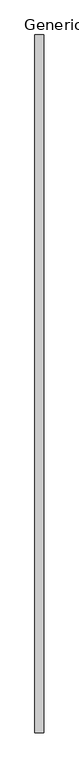
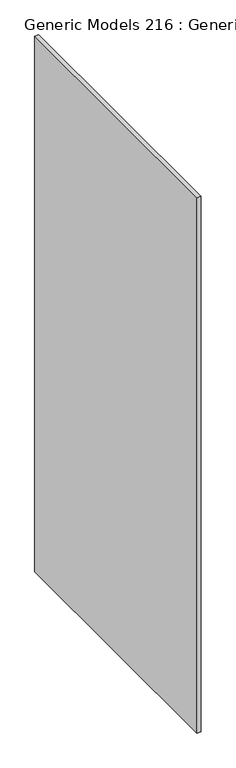
"""IFC4 building model written with IfcOpenShell, lengths in millimetres: proxy geometry, Generic Models 216 : Generic Models 1."""

import ifcopenshell
import ifcopenshell.guid

model = None  # the IFC model being written
_history = None  # IfcOwnerHistory: only IFC2X3 demands one
_inside = {}  # id of a spatial element -> (the spatial element, [elements in it])
_under = {}  # id of a project, library or spatial element -> (it, [spatial elements below it])
_declared = {}  # id of a project -> (the project, [libraries it declares])
_typed = {}  # id of a type object -> (the type object, [elements of that type])
_made_of = {}  # id of a material, layer set ... -> (it, [elements and type objects made of it])


def new_model(schema):
    """Start an empty IFC model of exactly this schema.

    Asked for "IFC4X3", IfcOpenShell would pick the latest addendum, in which some entities
    have other attributes; the version numbers below select the first issue.
    IFC2X3 requires an IfcOwnerHistory on every rooted entity: one is made here for all.
    """
    global model, _history
    if schema == "IFC4X3":
        model = ifcopenshell.file(schema_version=(4, 3, 0, 0))
    else:
        model = ifcopenshell.file(schema=schema)
    _inside.clear()
    _under.clear()
    _declared.clear()
    _typed.clear()
    _made_of.clear()
    _history = None
    if model.schema == "IFC2X3":
        org = make("IfcOrganization", Name="unknown")
        user = make(
            "IfcPersonAndOrganization",
            ThePerson=make("IfcPerson", FamilyName="unknown"),
            TheOrganization=org,
        )
        app = make(
            "IfcApplication",
            ApplicationDeveloper=org,
            Version="unknown",
            ApplicationFullName="unknown",
            ApplicationIdentifier="unknown",
        )
        _history = make(
            "IfcOwnerHistory",
            OwningUser=user,
            OwningApplication=app,
            ChangeAction="ADDED",
            CreationDate=0,
        )
    return model


def make(cls, **values):
    """One entity of the class cls with the attributes given. An attribute that is None is left unset."""
    return model.create_entity(
        cls, **{name: value for name, value in values.items() if value is not None}
    )


def rooted(cls, **values):
    """An entity with a GlobalId (a new one), such as an element, a storey or a relation."""
    return make(cls, GlobalId=ifcopenshell.guid.new(), OwnerHistory=_history, **values)


def si_unit(unit_type, name, prefix=None):
    """IfcSIUnit, for example si_unit("LENGTHUNIT", "METRE", prefix="MILLI")."""
    return make("IfcSIUnit", UnitType=unit_type, Prefix=prefix, Name=name)


def assignment(units):
    """IfcUnitAssignment: the units of a project."""
    return None if units is None else make("IfcUnitAssignment", Units=units)


def point(xyz):
    """IfcCartesianPoint."""
    return None if xyz is None else make("IfcCartesianPoint", Coordinates=xyz)


def direction(xyz):
    """IfcDirection."""
    return None if xyz is None else make("IfcDirection", DirectionRatios=xyz)


def frame(location, z_axis=None, x_axis=None):
    """IfcAxis2Placement3D, a coordinate frame: its origin and axes. An axis left out is left unset."""
    return make(
        "IfcAxis2Placement3D",
        Location=point(location),
        Axis=direction(z_axis),
        RefDirection=direction(x_axis),
    )


def origin():
    """The frame at (0, 0, 0) with its axes left unset."""
    return frame((0.0, 0.0, 0.0))


def place(relative_to, where):
    """IfcLocalPlacement: puts the frame where relative to a parent placement (None: the world)."""
    return make(
        "IfcLocalPlacement", PlacementRelTo=relative_to, RelativePlacement=where
    )


def context(
    kind, dimensions, precision=None, world=None, true_north=None, identifier=None
):
    """IfcGeometricRepresentationContext, for example the 3D "Model" context."""
    return make(
        "IfcGeometricRepresentationContext",
        ContextIdentifier=identifier,
        ContextType=kind,
        CoordinateSpaceDimension=dimensions,
        Precision=precision,
        WorldCoordinateSystem=world,
        TrueNorth=true_north,
    )


def project(units=None, contexts=None):
    """IfcProject with its units and contexts."""
    return rooted(
        "IfcProject",
        Name="project",
        RepresentationContexts=contexts,
        UnitsInContext=assignment(units),
    )


def spatial(cls, under=None, at=None, **own):
    """A site, building, storey or space (cls), placed at a placement, below another one or the project."""
    s = rooted(cls, ObjectPlacement=at, **own)
    if under is not None:
        _under.setdefault(under.id(), (under, []))[1].append(s)
    return s


def polyline(points):
    """IfcPolyline through the points."""
    return make("IfcPolyline", Points=[point(p) for p in points])


def outline(outer, holes=None, kind="AREA"):
    """IfcArbitraryClosedProfileDef: a profile drawn as a closed curve; with holes, ...WithVoids."""
    if holes is None:
        return make("IfcArbitraryClosedProfileDef", ProfileType=kind, OuterCurve=outer)
    return make(
        "IfcArbitraryProfileDefWithVoids",
        ProfileType=kind,
        OuterCurve=outer,
        InnerCurves=holes,
    )


def extrude(swept, where, along, depth):
    """IfcExtrudedAreaSolid: the profile swept, set in the frame where, extruded along a direction by depth."""
    return make(
        "IfcExtrudedAreaSolid",
        SweptArea=swept,
        Position=where,
        ExtrudedDirection=direction(along),
        Depth=depth,
    )


def shape(context_of_items, identifier, shape_type, items):
    """IfcShapeRepresentation: the items that make up one representation, for example the "Body"."""
    return make(
        "IfcShapeRepresentation",
        ContextOfItems=context_of_items,
        RepresentationIdentifier=identifier,
        RepresentationType=shape_type,
        Items=items,
    )


def source(mapping_origin, context_of_items, identifier, shape_type, items):
    """IfcRepresentationMap: a shape defined once, which mapped items show again and again."""
    return make(
        "IfcRepresentationMap",
        MappingOrigin=mapping_origin,
        MappedRepresentation=shape(context_of_items, identifier, shape_type, items),
    )


def transform(
    local_origin,
    x_axis=None,
    y_axis=None,
    z_axis=None,
    scale=None,
    scale2=None,
    scale3=None,
    uniform=True,
):
    """IfcCartesianTransformationOperator3D, or its non-uniform kind. x_axis, y_axis, z_axis: its Axis1, 2, 3."""
    if uniform:
        return make(
            "IfcCartesianTransformationOperator3D",
            Axis1=direction(x_axis),
            Axis2=direction(y_axis),
            LocalOrigin=point(local_origin),
            Scale=scale,
            Axis3=direction(z_axis),
        )
    return make(
        "IfcCartesianTransformationOperator3DnonUniform",
        Axis1=direction(x_axis),
        Axis2=direction(y_axis),
        LocalOrigin=point(local_origin),
        Scale=scale,
        Axis3=direction(z_axis),
        Scale2=scale2,
        Scale3=scale3,
    )


def mapped(mapping_source, mapping_target):
    """IfcMappedItem: shows the shape of a source again, moved by a transform."""
    return make(
        "IfcMappedItem", MappingSource=mapping_source, MappingTarget=mapping_target
    )


def made_of(thing, what):
    """Note that an element or type object is made of a material, layer set ...; save() writes the relation."""
    if what is not None:
        _made_of.setdefault(what.id(), (what, []))[1].append(thing)
    return thing


def element(
    cls,
    number,
    at=None,
    inside=None,
    cuts=None,
    type_object=None,
    material=None,
    context=None,
    identifier="Body",
    shape_type=None,
    held_by="IfcProductDefinitionShape",
    body=None,
    shapes=None,
    **own,
):
    """One element of the class cls, such as IfcWall. Its Tag is "e" and its number.

    at: its placement. inside: the storey or other place that contains it. cuts: it is an
    opening in that element (IfcRelVoidsElement). A single representation is given by context,
    identifier, shape_type and body (its items); several are given by shapes. held_by: the class
    of the entity that holds the representations. save() writes the other relations.
    """
    e = rooted(cls, Tag="e%d" % number, ObjectPlacement=at, **own)
    if body is not None:
        shapes = [shape(context, identifier, shape_type, body)]
    if shapes is not None:
        e.Representation = make(held_by, Representations=shapes)
    if inside is not None:
        _inside.setdefault(inside.id(), (inside, []))[1].append(e)
    if cuts is not None:
        rooted(
            "IfcRelVoidsElement", RelatingBuildingElement=cuts, RelatedOpeningElement=e
        )
    if type_object is not None:
        _typed.setdefault(type_object.id(), (type_object, []))[1].append(e)
    return made_of(e, material)


def aggregate(whole, parts):
    """IfcRelAggregates: a whole, such as a stair, and the parts it consists of."""
    return rooted("IfcRelAggregates", RelatingObject=whole, RelatedObjects=parts)


def save(model, path):
    """Write the relations noted so far, then the file.

    IfcRelAggregates (storeys below a building ...), IfcRelContainedInSpatialStructure (elements
    in a storey), IfcRelDefinesByType, IfcRelAssociatesMaterial and IfcRelDeclares: one each for
    every whole, place, type object, material and project.
    """
    for whole, parts in _under.values():
        aggregate(whole, parts)
    for where, things in _inside.values():
        rooted(
            "IfcRelContainedInSpatialStructure",
            RelatedElements=things,
            RelatingStructure=where,
        )
    for kind, things in _typed.values():
        rooted("IfcRelDefinesByType", RelatedObjects=things, RelatingType=kind)
    for what, things in _made_of.values():
        rooted("IfcRelAssociatesMaterial", RelatedObjects=things, RelatingMaterial=what)
    for by, libraries in _declared.values():
        rooted("IfcRelDeclares", RelatingContext=by, RelatedDefinitions=libraries)
    model.write(path)


def generic_models_216_generic_models_1_e9c984b2(model_context):
    return source(origin(), model_context, "Body", "SweptSolid", [
        extrude(outline(polyline([(48580.675, 1219.2), (48580.675, 0.0), (48564.8, 0.0), (48564.8, 1219.2), (48580.675, 1219.2)])), frame((0.0, 0.0, 3054.35), z_axis=(0.0, 0.0, 1.0), x_axis=(1.0, 0.0, 0.0)), (0.0, 0.0, 1.0), 2451.1),
    ])


if __name__ == "__main__":
    model = new_model("IFC4")
    model_context = context("Model", 3, world=origin())
    ifc_project = project(units=[si_unit("LENGTHUNIT", "METRE", prefix="MILLI")], contexts=[model_context])
    site = spatial("IfcSite", under=ifc_project)
    building = spatial("IfcBuilding", under=site)
    placement = place(None, origin())
    generic_models_216_generic_models_1_shape = generic_models_216_generic_models_1_e9c984b2(model_context)
    element("IfcBuildingElementProxy", 1, Name="Generic Models 216 : Generic Models 1", ObjectType="Generic Models 216 : Generic Models 1", at=placement, inside=building, context=model_context, shape_type="MappedRepresentation", body=[
        mapped(generic_models_216_generic_models_1_shape, transform((0.0, 0.0, 0.0), x_axis=(1.0, 0.0, 0.0), y_axis=(0.0, 1.0, 0.0), z_axis=(0.0, 0.0, 1.0))),
    ])
    save(model, "model.ifc")

# Revit data of these elements
# Element 1 (IfcBuildingElementProxy, "Generic Models 216 : Generic Models 1")
#   Materials on its faces: "GYP. BD (SEE 'WALL TAG' & 'LAYER MATERIAL SCHEDULE' FOR DETAILS)"
# Materials
#   "GYP. BD (SEE 'WALL TAG' & 'LAYER MATERIAL SCHEDULE' FOR DETAILS)": class "Generic", colour RGB 237 236 233, transparency 0, Description = "Gypsum Wall Board", Cost = 0
